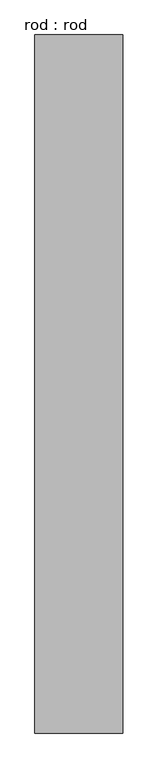
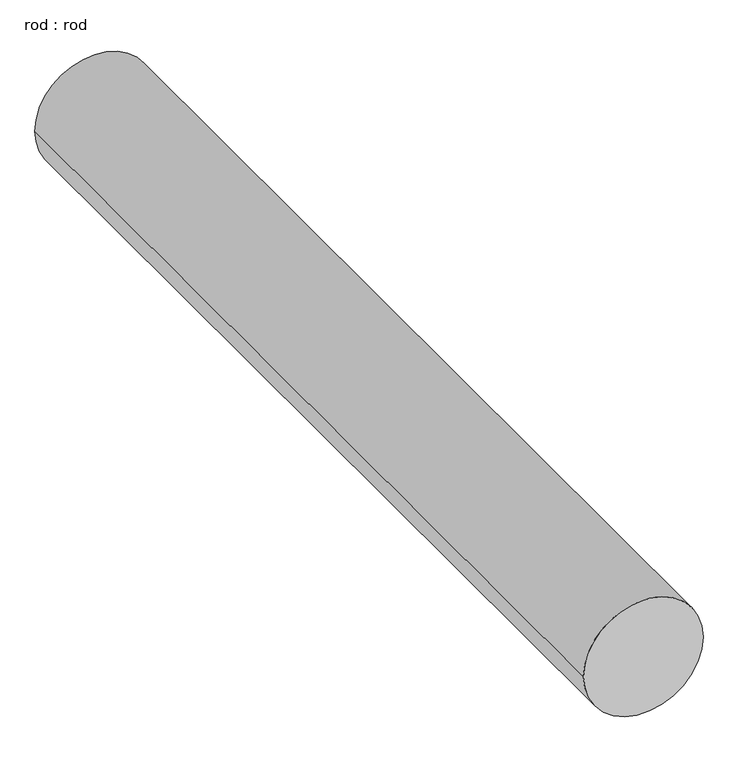
"""IFC4 building model written with IfcOpenShell, lengths in millimetres: proxy geometry, rod : rod."""

from ifc_helpers import new_model, si_unit, point, frame, frame_2d, origin, place, context, project, spatial, circle_curve, trimmed, segment, composite_curve, outline, extrude, source, transform, mapped, element, save


def rod_rod_44d3c6fe(model_context):
    return source(origin(), model_context, "Body", "SweptSolid", [
        extrude(outline(composite_curve([segment(trimmed(circle_curve(frame_2d((0.0108462, 0.0)), 200.0), [point((0.0108462, 200.0))], [point((0.0108462, -200.0))], False, "CARTESIAN"), True, "CONTINUOUS"), segment(trimmed(circle_curve(frame_2d((0.0108462, 0.0)), 200.0), [point((0.0108462, -200.0))], [point((0.0108462, 200.0))], False, "CARTESIAN"), True, "CONTINUOUS")], self_intersect=False)), frame((0.0, 2502.7286153, 0.0), z_axis=(0.0, 1.0, 0.0), x_axis=(0.0, 0.0, 1.0)), (0.0, 0.0, 1.0), 3180.0),
    ])


if __name__ == "__main__":
    model = new_model("IFC4")
    model_context = context("Model", 3, world=origin())
    ifc_project = project(units=[si_unit("LENGTHUNIT", "METRE", prefix="MILLI")], contexts=[model_context])
    site = spatial("IfcSite", under=ifc_project)
    building = spatial("IfcBuilding", under=site)
    placement = place(None, origin())
    rod_rod_shape = rod_rod_44d3c6fe(model_context)
    element("IfcBuildingElementProxy", 1, Name="rod : rod", ObjectType="rod : rod", at=placement, inside=building, context=model_context, shape_type="MappedRepresentation", body=[
        mapped(rod_rod_shape, transform((0.0, 0.0, 0.0), x_axis=(1.0, 0.0, 0.0), y_axis=(0.0, 1.0, 0.0), z_axis=(0.0, 0.0, 1.0))),
    ])
    save(model, "model.ifc")

# Revit data of these elements
# Type "rod : rod"
#   Default Elevation = 0
